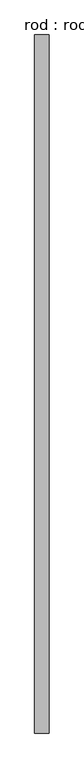
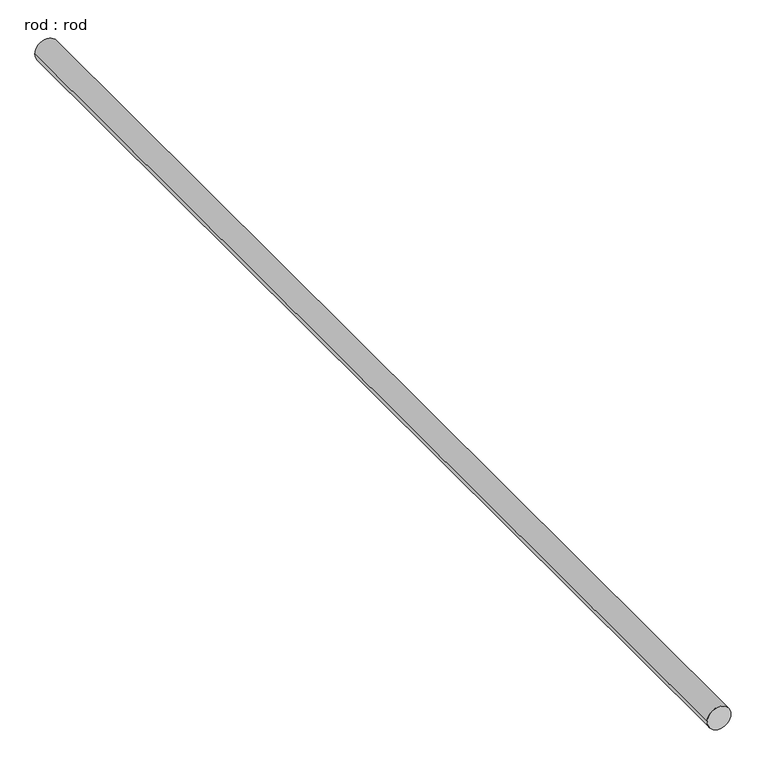
"""IFC4 building model written with IfcOpenShell, lengths in millimetres: proxy geometry, rod : rod."""

from ifc_helpers import new_model, si_unit, point, frame, frame_2d, origin, place, context, project, spatial, circle_curve, trimmed, segment, composite_curve, outline, extrude, source, transform, mapped, element, save


def rod_rod_c3f67fb2(model_context):
    return source(origin(), model_context, "Body", "SweptSolid", [
        extrude(outline(composite_curve([segment(trimmed(circle_curve(frame_2d((0.0108462, 0.0)), 200.0), [point((0.0108462, 200.0))], [point((0.0108462, -200.0))], False, "CARTESIAN"), True, "CONTINUOUS"), segment(trimmed(circle_curve(frame_2d((0.0108462, 0.0)), 200.0), [point((0.0108462, -200.0))], [point((0.0108462, 200.0))], False, "CARTESIAN"), True, "CONTINUOUS")], self_intersect=False)), frame((0.0, -5719.7713847, 0.0), z_axis=(0.0, 1.0, 0.0), x_axis=(0.0, 0.0, 1.0)), (0.0, 0.0, 1.0), 19625.0),
    ])


if __name__ == "__main__":
    model = new_model("IFC4")
    model_context = context("Model", 3, world=origin())
    ifc_project = project(units=[si_unit("LENGTHUNIT", "METRE", prefix="MILLI")], contexts=[model_context])
    site = spatial("IfcSite", under=ifc_project)
    building = spatial("IfcBuilding", under=site)
    placement = place(None, origin())
    rod_rod_shape = rod_rod_c3f67fb2(model_context)
    element("IfcBuildingElementProxy", 1, Name="rod : rod", ObjectType="rod : rod", at=placement, inside=building, context=model_context, shape_type="MappedRepresentation", body=[
        mapped(rod_rod_shape, transform((0.0, 0.0, 0.0), x_axis=(1.0, 0.0, 0.0), y_axis=(0.0, 1.0, 0.0), z_axis=(0.0, 0.0, 1.0))),
    ])
    save(model, "model.ifc")

# Revit data of these elements
# Type "rod : rod"
#   Default Elevation = 0
